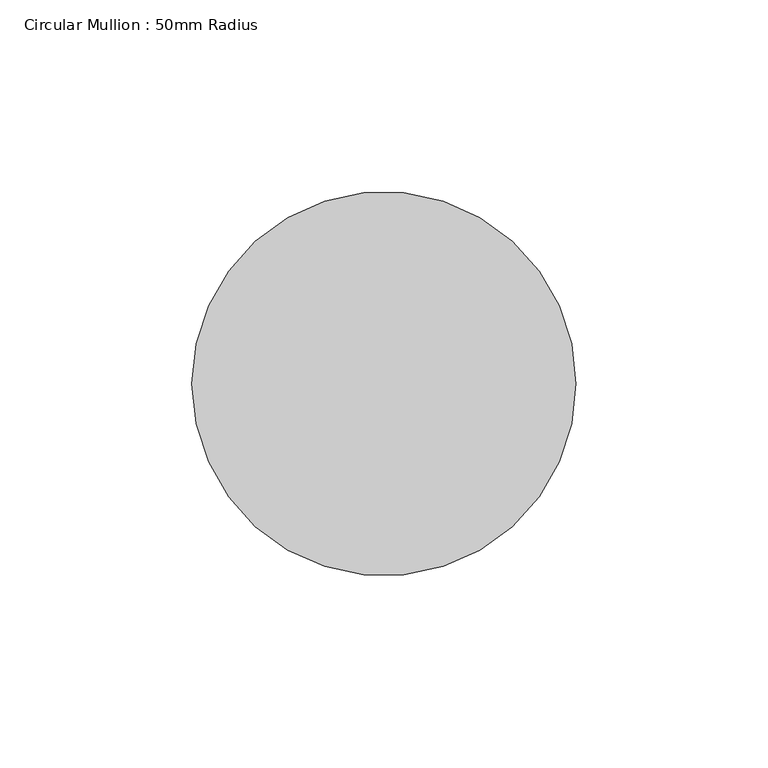
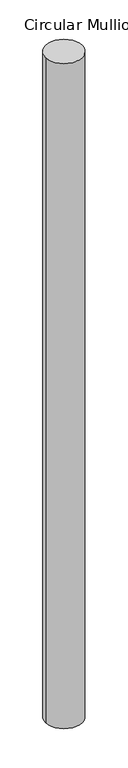
"""IFC4 building model written with IfcOpenShell, lengths in millimetres: member geometry, Circular Mullion : 50mm Radius."""

from ifc_helpers import new_model, si_unit, point, frame, frame_2d, origin, place, context, project, spatial, circle_curve, trimmed, segment, composite_curve, outline, extrude, source, transform, mapped, element, save


def circular_mullion_50mm_radius_a7901719(model_context):
    return source(origin(), model_context, "Body", "SweptSolid", [
        extrude(outline(composite_curve([segment(trimmed(circle_curve(frame_2d((-50.0, 0.0)), 50.0), [point((0.0, 0.0))], [point((-100.0, 0.0))], False, "CARTESIAN"), True, "CONTINUOUS"), segment(trimmed(circle_curve(frame_2d((-50.0, 0.0)), 50.0), [point((-100.0, 0.0))], [point((0.0, 0.0))], False, "CARTESIAN"), True, "CONTINUOUS")], self_intersect=False)), frame((0.0, 0.0, -1913.5592469), z_axis=(0.0, 0.0, 1.0), x_axis=(1.0, 0.0, 0.0)), (0.0, 0.0, 1.0), 1913.5592469),
    ])


if __name__ == "__main__":
    model = new_model("IFC4")
    model_context = context("Model", 3, world=origin())
    ifc_project = project(units=[si_unit("LENGTHUNIT", "METRE", prefix="MILLI")], contexts=[model_context])
    site = spatial("IfcSite", under=ifc_project)
    building = spatial("IfcBuilding", under=site)
    placement = place(None, origin())
    circular_mullion_50mm_radius_shape = circular_mullion_50mm_radius_a7901719(model_context)
    element("IfcMember", 1, ObjectType="Circular Mullion : 50mm Radius", at=placement, inside=building, context=model_context, shape_type="MappedRepresentation", body=[
        mapped(circular_mullion_50mm_radius_shape, transform((0.0, 0.0, 0.0), x_axis=(1.0, 0.0, 0.0), y_axis=(0.0, 1.0, 0.0), z_axis=(0.0, 0.0, 1.0))),
    ])
    save(model, "model.ifc")

# Revit data of these elements
# Type "Circular Mullion : 50mm Radius"
#   built-in parameter 1007350 = 0.164042 (stored number, unit not read)
# Element 1 (IfcMember, "Circular Mullion : 50mm Radius")
#   Materials on its faces: "Aluminium"
# Materials
#   "Aluminium": class "Metal", colour RGB 247 247 247, transparency 0, Description = "Aluminium 6061", Cost = 0
